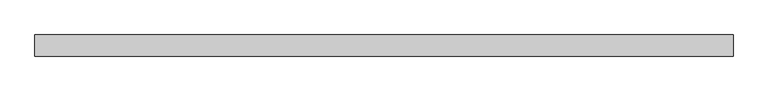
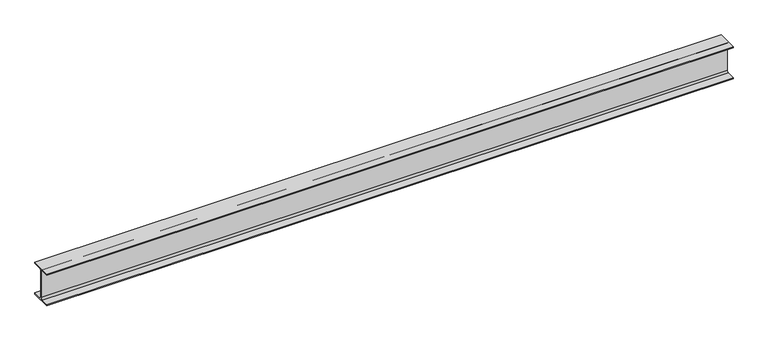
"""IFC4 building model written with IfcOpenShell, lengths in millimetres: beam geometry, 0912_Steel Framing_H-KSD3502 : H_SB_ASB_H-488x300x11x18."""

from ifc_helpers import new_model, si_unit, point, frame, frame_2d, origin, place, context, project, spatial, polyline, circle_curve, trimmed, segment, composite_curve, outline, extrude, source, transform, mapped, element, save


def beam_2afad9e3(model_context):
    return source(origin(), model_context, "Body", "SweptSolid", [
        extrude(outline(composite_curve([segment(polyline([(150.0, -226.0), (150.0, -244.0), (-150.0, -244.0), (-150.0, -226.0), (-31.5, -226.0)]), True, "CONTINUOUS"), segment(trimmed(circle_curve(frame_2d((-31.5, -200.0)), 26.0), [point((-31.5, -226.0))], [point((-5.5, -200.0))], True, "CARTESIAN"), True, "CONTINUOUS"), segment(polyline([(-5.5, -200.0), (-5.5, 200.0)]), True, "CONTINUOUS"), segment(trimmed(circle_curve(frame_2d((-31.5, 200.0)), 26.0), [point((-5.5, 200.0))], [point((-31.5, 226.0))], True, "CARTESIAN"), True, "CONTINUOUS"), segment(polyline([(-31.5, 226.0), (-150.0, 226.0), (-150.0, 244.0), (150.0, 244.0), (150.0, 226.0), (31.5, 226.0)]), True, "CONTINUOUS"), segment(trimmed(circle_curve(frame_2d((31.5, 200.0)), 26.0), [point((31.5, 226.0))], [point((5.5, 200.0))], True, "CARTESIAN"), True, "CONTINUOUS"), segment(polyline([(5.5, 200.0), (5.5, -200.0)]), True, "CONTINUOUS"), segment(trimmed(circle_curve(frame_2d((31.5, -200.0)), 26.0), [point((5.5, -200.0))], [point((31.5, -226.0))], True, "CARTESIAN"), True, "CONTINUOUS"), segment(polyline([(31.5, -226.0), (150.0, -226.0)]), True, "CONTINUOUS")], self_intersect=False)), frame((-4962.3, 0.0, 0.0), z_axis=(1.0, 0.0, 0.0), x_axis=(0.0, 1.0, 0.0)), (0.0, 0.0, 1.0), 9924.6),
    ])


if __name__ == "__main__":
    model = new_model("IFC4")
    model_context = context("Model", 3, world=origin())
    ifc_project = project(units=[si_unit("LENGTHUNIT", "METRE", prefix="MILLI")], contexts=[model_context])
    site = spatial("IfcSite", under=ifc_project)
    building = spatial("IfcBuilding", under=site)
    placement = place(None, origin())
    beam_shape = beam_2afad9e3(model_context)
    element("IfcBeam", 1, ObjectType="0912_Steel Framing_H-KSD3502 : H_SB_ASB_H-488x300x11x18", at=placement, inside=building, context=model_context, shape_type="MappedRepresentation", body=[
        mapped(beam_shape, transform((0.0, 0.0, 0.0), x_axis=(1.0, 0.0, 0.0), y_axis=(0.0, 1.0, 0.0), z_axis=(0.0, 0.0, 1.0))),
    ])
    save(model, "model.ifc")

# Revit data of these elements
# Type "0912_Steel Framing_H-KSD3502 : H_SB_ASB_H-488x300x11x18"
#   H_WM Code_1 = "S01AA001-00001 | Main Steel Structure Fabrication Work | Shelter/Building | Heavy Steel - Standard (Weight≥90KG/M) | Material: (   )"
#   H_WM Code_2 = "S03AA027-00001 | Main Steel Structure Erection Work | Shelter/Building | Heavy Steel (Weight≥90KG/M) | Material: (   )"
#   H_WM Code_3 = "S01AA010-00001 | Main Steel Structure Fabrication Work | Shelter/Building | Steel Painting/Coating | for Non-Fireproofed Steel Surface, Surface Preparation, Primer, Second & Final Coat | Material: (   )"
#   H_Q'ty Cal Type Tag = "SB-Q2"
#   Width = 30.0 cm
#   Web Thickness = 1.1 cm
#   Web Fillet = 2.6 cm
#   Warping Constant = 4470000.0 cm⁶
#   W = 0
#   Torsional Moment of Inertia = 137.492 cm⁴
#   Section Area = 163.5 cm²
#   Plastic Modulus weak axis = 830.0 cm³
#   Plastic Modulus strong axis = 3230.0 cm³
#   Perimeter = 2.11 m²/m
#   Nominal Weight = 128.00 kgf/m
#   Moment of Inertia weak axis = 8110.00 cm⁴
#   Moment of Inertia strong axis = 71000.00 cm⁴
#   Height = 48.8 cm
#   Flange Thickness = 1.8 cm
#   Elastic Modulus weak axis = 541.0 cm³
#   Elastic Modulus strong axis = 2910.0 cm³
#   Centroid Vertical = 24.4 cm
#   Centroid Horizontal = 15.0 cm
#   Ix = 710000000
#   Length [instance default] = 1.5240 m
#   Zx = 3230000
#   b = 0.3000 m
#   h = 0.4880 m
#   r = 0.0260 m
#   s = 0.0110 m
#   t = 0.0180 m
#   A = 0.01635 m²
#   Structural Material [instance default] = Steel, 45-345
#   Assembly Code = ""
# Element 1 (IfcBeam, "0912_Steel Framing_H-KSD3502 : H_SB_ASB_H-488x300x11x18")
#   Structural Material = none
# Materials
#   "Steel, 45-345": class "Metal", colour RGB 189 187 185, transparency 0, Description = "Steel 345 MPa", Cost = 0
